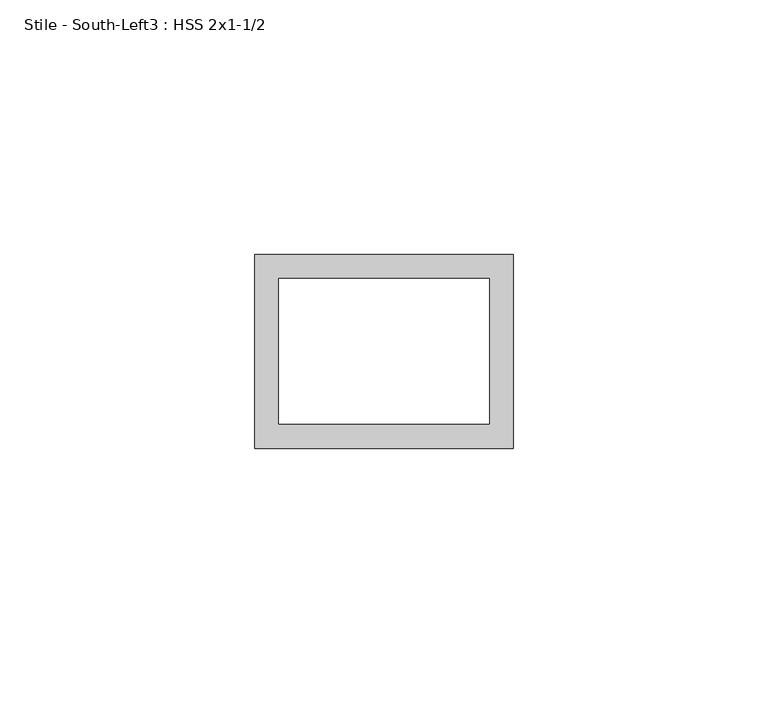
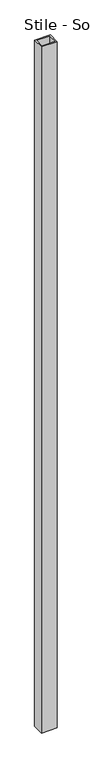
"""IFC4 building model written with IfcOpenShell, lengths in millimetres: proxy geometry, Stile - South-Left3 : HSS 2x1-1/2."""

from ifc_helpers import new_model, si_unit, frame, origin, place, context, project, spatial, polyline, outline, extrude, source, transform, mapped, element, save


def stile_south_left3_hss_2x1_1_2_18bcf153(model_context):
    return source(origin(), model_context, "Body", "SweptSolid", [
        extrude(outline(polyline([(587365.8934739, -535207.9163841), (587416.6934739, -535207.9163841), (587416.6934739, -535246.0163841), (587365.8934739, -535246.0163841), (587365.8934739, -535207.9163841)]), holes=[polyline([(587370.6559739, -535212.6788841), (587370.6559739, -535241.2538841), (587411.9309739, -535241.2538841), (587411.9309739, -535212.6788841), (587370.6559739, -535212.6788841)])]), frame((0.0, 0.0, 50.8), z_axis=(0.0, 0.0, 1.0), x_axis=(1.0, 0.0, 0.0)), (0.0, 0.0, 1.0), 2349.5),
    ])


if __name__ == "__main__":
    model = new_model("IFC4")
    model_context = context("Model", 3, world=origin())
    ifc_project = project(units=[si_unit("LENGTHUNIT", "METRE", prefix="MILLI")], contexts=[model_context])
    site = spatial("IfcSite", under=ifc_project)
    building = spatial("IfcBuilding", under=site)
    placement = place(None, origin())
    stile_south_left3_hss_2x1_1_2_shape = stile_south_left3_hss_2x1_1_2_18bcf153(model_context)
    element("IfcBuildingElementProxy", 1, Name="Stile - South-Left3 : HSS 2x1-1/2", ObjectType="Stile - South-Left3 : HSS 2x1-1/2", at=placement, inside=building, context=model_context, shape_type="MappedRepresentation", body=[
        mapped(stile_south_left3_hss_2x1_1_2_shape, transform((0.0, 0.0, 0.0), x_axis=(1.0, 0.0, 0.0), y_axis=(0.0, 1.0, 0.0), z_axis=(0.0, 0.0, 1.0))),
    ])
    save(model, "model.ifc")

# Revit data of these elements
# Element 1 (IfcBuildingElementProxy, "Stile - South-Left3 : HSS 2x1-1/2")
#   Materials on its faces: "1-1/2\"X2\" GALV. STL HSS TUBING"
# Materials
#   "1-1/2\"X2\" GALV. STL HSS TUBING": class "Generic", colour RGB 211 211 207, transparency 0, Cost = 0
